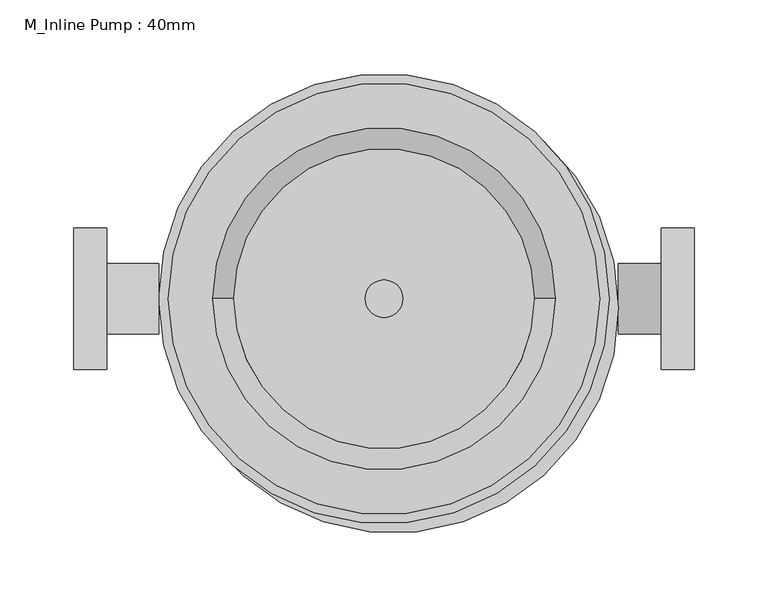
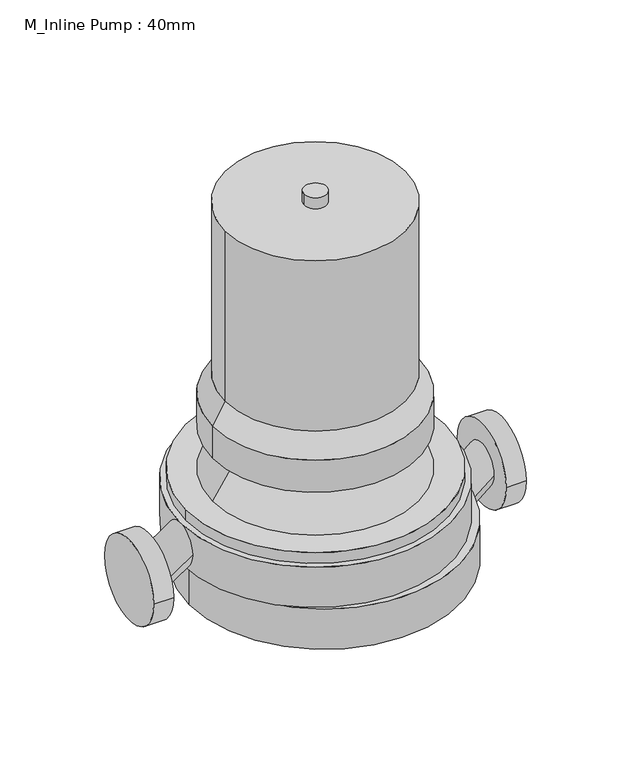
"""IFC4 building model written with IfcOpenShell, lengths in millimetres: proxy geometry, M_Inline Pump : 40mm."""

from ifc_helpers import new_model, si_unit, point, frame, frame_2d, origin, origin_with_axes, origin_2d, place, context, project, spatial, polyline, circle_curve, trimmed, segment, composite_curve, outline, extrude, source, transform, mapped, element, save
from ifc_brep_helpers import plane_surface, revolved_surface, extruded_surface, advanced_brep


def m_inline_pump_40mm_c178c80e(model_context):
    return source(origin(), model_context, "Body", "SolidModel", [
        advanced_brep(
        [(158.75, -24.0, -24.0), (158.75, 24.0, -24.0), (187.7, -24.0, 0.0), (187.7, 24.0, 0.0)],
        [
            (0, 1, circle_curve(frame((158.75, 0.0, -24.0), z_axis=(-1.0, 0.0, 0.0), x_axis=(0.0, 1.0, 0.0)), 24.0)),
            (1, 0, circle_curve(frame((158.75, 0.0, -24.0), z_axis=(-1.0, 0.0, 0.0), x_axis=(0.0, 1.0, 0.0)), 24.0)),
            (2, 3, circle_curve(frame((187.7, 0.0, 0.0), z_axis=(1.0, 0.0, 0.0), x_axis=(0.0, 1.0, 0.0)), 24.0)),
            (3, 2, circle_curve(frame((187.7, 0.0, 0.0), z_axis=(1.0, 0.0, 0.0), x_axis=(0.0, 1.0, 0.0)), 24.0)),
            (3, 1),
            (0, 2),
        ],
        [
            plane_surface(frame((158.75, 0.0, -24.0), z_axis=(-1.0, 0.0, 0.0), x_axis=(0.0, 0.0, -1.0))),
            plane_surface(frame((187.7, 0.0, 0.0), z_axis=(1.0, 0.0, 0.0), x_axis=(0.0, 0.0, -1.0))),
            extruded_surface(trimmed(circle_curve(frame((187.7, 0.0, 0.0), z_axis=(-1.0, 0.0, 0.0), x_axis=(0.0, 1.0, 0.0)), 24.0), [point((187.7, -24.0, 0.0))], [point((187.7, 24.0, 0.0))], True, "CARTESIAN"), (-28.94999999999999, 0.0, -24.0), 37.604554245463405),
            extruded_surface(trimmed(circle_curve(frame((187.7, 0.0, 0.0), z_axis=(-1.0, 0.0, 0.0), x_axis=(0.0, 1.0, 0.0)), 24.0), [point((187.7, 24.0, 0.0))], [point((187.7, -24.0, 0.0))], True, "CARTESIAN"), (-28.94999999999999, 0.0, -24.0), 37.604554245463405),
        ],
        [
            (0, [[1, 2]]),
            (1, [[3, 4]]),
            (2, [[-4, 5, -1, 6]]),
            (3, [[-3, -6, -2, -5]]),
        ],
    ),
        extrude(outline(composite_curve([segment(trimmed(circle_curve(origin_2d(), 48.0), [point((-48.0, 0.0))], [point((48.0, 0.0))], False, "CARTESIAN"), True, "CONTINUOUS"), segment(trimmed(circle_curve(origin_2d(), 48.0), [point((48.0, 0.0))], [point((-48.0, 0.0))], False, "CARTESIAN"), True, "CONTINUOUS")], self_intersect=False)), frame((187.7, 0.0, 0.0), z_axis=(1.0, 0.0, 0.0), x_axis=(0.0, 1.0, 0.0)), (0.0, 0.0, 1.0), 22.3),
        advanced_brep(
        [(-152.4, -24.0, 24.0), (-152.4, 24.0, 24.0), (-187.7, -24.0, 0.0), (-187.7, 24.0, 0.0)],
        [
            (0, 1, circle_curve(frame((-152.4, 0.0, 24.0), z_axis=(1.0, 0.0, 0.0), x_axis=(0.0, 1.0, 0.0)), 24.0)),
            (1, 0, circle_curve(frame((-152.4, 0.0, 24.0), z_axis=(1.0, 0.0, 0.0), x_axis=(0.0, 1.0, 0.0)), 24.0)),
            (2, 3, circle_curve(frame((-187.7, 0.0, 0.0), z_axis=(-1.0, 0.0, 0.0), x_axis=(0.0, 1.0, 0.0)), 24.0)),
            (3, 2, circle_curve(frame((-187.7, 0.0, 0.0), z_axis=(-1.0, 0.0, 0.0), x_axis=(0.0, 1.0, 0.0)), 24.0)),
            (3, 1),
            (0, 2),
        ],
        [
            plane_surface(frame((-152.4, 0.0, 24.0), z_axis=(1.0, 0.0, 0.0), x_axis=(0.0, 0.0, -1.0))),
            plane_surface(frame((-187.7, 0.0, 0.0), z_axis=(-1.0, 0.0, 0.0), x_axis=(0.0, 0.0, -1.0))),
            extruded_surface(trimmed(circle_curve(frame((-187.7, 0.0, 0.0), z_axis=(1.0, 0.0, 0.0), x_axis=(0.0, 1.0, 0.0)), 24.0), [point((-187.7, -24.0, 0.0))], [point((-187.7, 24.0, 0.0))], True, "CARTESIAN"), (35.29999999999998, 0.0, 24.0), 42.68594616498501),
            extruded_surface(trimmed(circle_curve(frame((-187.7, 0.0, 0.0), z_axis=(1.0, 0.0, 0.0), x_axis=(0.0, 1.0, 0.0)), 24.0), [point((-187.7, 24.0, 0.0))], [point((-187.7, -24.0, 0.0))], True, "CARTESIAN"), (35.29999999999998, 0.0, 24.0), 42.68594616498501),
        ],
        [
            (0, [[1, 2]]),
            (1, [[3, 4]]),
            (2, [[-4, 5, -1, 6]]),
            (3, [[-3, -6, -2, -5]]),
        ],
    ),
        extrude(outline(composite_curve([segment(trimmed(circle_curve(origin_2d(), 48.0), [point((-48.0, 0.0))], [point((48.0, 0.0))], False, "CARTESIAN"), True, "CONTINUOUS"), segment(trimmed(circle_curve(origin_2d(), 48.0), [point((48.0, 0.0))], [point((-48.0, 0.0))], False, "CARTESIAN"), True, "CONTINUOUS")], self_intersect=False)), frame((-210.0, 0.0, 0.0), z_axis=(1.0, 0.0, 0.0), x_axis=(0.0, 1.0, 0.0)), (0.0, 0.0, 1.0), 22.3),
        extrude(outline(composite_curve([segment(trimmed(circle_curve(origin_2d(), 12.7), [point((-12.7, 0.0))], [point((12.7, 0.0))], False, "CARTESIAN"), True, "CONTINUOUS"), segment(trimmed(circle_curve(origin_2d(), 12.7), [point((12.7, 0.0))], [point((-12.7, 0.0))], False, "CARTESIAN"), True, "CONTINUOUS")], self_intersect=False)), frame((0.0, 0.0, 378.0), z_axis=(0.0, 0.0, 1.0), x_axis=(1.0, 0.0, 0.0)), (0.0, 0.0, 1.0), 13.0),
        extrude(outline(composite_curve([segment(trimmed(circle_curve(origin_2d(), 152.4), [point((-152.4, 0.0))], [point((152.4, 0.0))], False, "CARTESIAN"), True, "CONTINUOUS"), segment(trimmed(circle_curve(origin_2d(), 152.4), [point((152.4, 0.0))], [point((-152.4, 0.0))], False, "CARTESIAN"), True, "CONTINUOUS")], self_intersect=False)), origin_with_axes(), (0.0, 0.0, 1.0), 48.0),
        extrude(outline(composite_curve([segment(trimmed(circle_curve(frame_2d((6.35, -6.35)), 152.4), [point((-146.05, -6.35))], [point((158.75, -6.35))], False, "CARTESIAN"), True, "CONTINUOUS"), segment(trimmed(circle_curve(frame_2d((6.35, -6.35)), 152.4), [point((158.75, -6.35))], [point((-146.05, -6.35))], False, "CARTESIAN"), True, "CONTINUOUS")], self_intersect=False)), frame((0.0, 0.0, -48.0), z_axis=(0.0, 0.0, 1.0), x_axis=(1.0, 0.0, 0.0)), (0.0, 0.0, 1.0), 48.0),
        extrude(outline(composite_curve([segment(trimmed(circle_curve(origin_2d(), 38.1), [point((-38.1, 0.0))], [point((38.1, 0.0))], False, "CARTESIAN"), True, "CONTINUOUS"), segment(trimmed(circle_curve(origin_2d(), 38.1), [point((38.1, 0.0))], [point((-38.1, 0.0))], False, "CARTESIAN"), True, "CONTINUOUS")], self_intersect=False)), frame((0.0, 0.0, -60.7198438), z_axis=(0.0, 0.0, 1.0), x_axis=(1.0, 0.0, 0.0)), (0.0, 0.0, 1.0), 12.7198438),
        extrude(outline(composite_curve([segment(trimmed(circle_curve(origin_2d(), 12.7), [point((-12.7, 0.0))], [point((12.7, 0.0))], False, "CARTESIAN"), True, "CONTINUOUS"), segment(trimmed(circle_curve(origin_2d(), 12.7), [point((12.7, 0.0))], [point((-12.7, 0.0))], False, "CARTESIAN"), True, "CONTINUOUS")], self_intersect=False)), frame((0.0, 0.0, -67.0698438), z_axis=(0.0, 0.0, 1.0), x_axis=(1.0, 0.0, 0.0)), (0.0, 0.0, 1.0), 6.35),
        extrude(outline(composite_curve([segment(trimmed(circle_curve(origin_2d(), 101.6), [point((-101.6, 0.0))], [point((101.6, 0.0))], False, "CARTESIAN"), True, "CONTINUOUS"), segment(trimmed(circle_curve(origin_2d(), 101.6), [point((101.6, 0.0))], [point((-101.6, 0.0))], False, "CARTESIAN"), True, "CONTINUOUS")], self_intersect=False)), frame((0.0, 0.0, 175.0), z_axis=(0.0, 0.0, 1.0), x_axis=(1.0, 0.0, 0.0)), (0.0, 0.0, 1.0), 203.0),
        advanced_brep(
        [(-101.6, 0.0, 175.0), (101.6, 0.0, 175.0), (-115.8875, 0.0, 150.0), (115.8875, 0.0, 150.0)],
        [
            (0, 1, circle_curve(frame((0.0, 0.0, 175.0), z_axis=(0.0, 0.0, 1.0), x_axis=(-1.0, 0.0, 0.0)), 101.6)),
            (1, 0, circle_curve(frame((0.0, 0.0, 175.0), z_axis=(0.0, 0.0, 1.0), x_axis=(1.0, 0.0, 0.0)), 101.6)),
            (2, 3, circle_curve(frame((0.0, 0.0, 150.0), z_axis=(0.0, 0.0, -1.0), x_axis=(1.0, 0.0, 0.0)), 115.8875)),
            (3, 2, circle_curve(frame((0.0, 0.0, 150.0), z_axis=(0.0, 0.0, -1.0), x_axis=(-1.0, 0.0, 0.0)), 115.8875)),
            (3, 1),
            (0, 2),
        ],
        [
            plane_surface(frame((0.0, 0.0, 175.0), z_axis=(0.0, 0.0, 1.0), x_axis=(0.0, -1.0, 0.0))),
            plane_surface(frame((0.0, 0.0, 150.0), z_axis=(0.0, 0.0, -1.0), x_axis=(0.0, -1.0, 0.0))),
            revolved_surface(polyline([(-101.60000000156576, 0.0, 175.0), (-115.8875, 0.0, 150.0)]), (0.0, 0.0, 352.7777778), (0.0, 0.0, -1.0)),
            revolved_surface(polyline([(101.60000000156576, 0.0, 175.0), (115.8875, 0.0, 150.0)]), (0.0, 0.0, 352.7777778), (0.0, 0.0, -1.0)),
        ],
        [
            (0, [[1, 2]]),
            (1, [[3, 4]]),
            (2, [[-4, 5, -1, 6]]),
            (3, [[-3, -6, -2, -5]]),
        ],
    ),
        extrude(outline(composite_curve([segment(trimmed(circle_curve(origin_2d(), 115.8875), [point((-115.8875, 0.0))], [point((115.8875, 0.0))], False, "CARTESIAN"), True, "CONTINUOUS"), segment(trimmed(circle_curve(origin_2d(), 115.8875), [point((115.8875, 0.0))], [point((-115.8875, 0.0))], False, "CARTESIAN"), True, "CONTINUOUS")], self_intersect=False)), frame((0.0, 0.0, 112.0), z_axis=(0.0, 0.0, 1.0), x_axis=(1.0, 0.0, 0.0)), (0.0, 0.0, 1.0), 38.0),
        advanced_brep(
        [(-82.55, 0.0, 112.0), (82.55, 0.0, 112.0), (-115.8875, 0.0, 61.0), (115.8875, 0.0, 61.0)],
        [
            (0, 1, circle_curve(frame((0.0, 0.0, 112.0), z_axis=(0.0, 0.0, 1.0), x_axis=(-1.0, 0.0, 0.0)), 82.55)),
            (1, 0, circle_curve(frame((0.0, 0.0, 112.0), z_axis=(0.0, 0.0, 1.0), x_axis=(1.0, 0.0, 0.0)), 82.55)),
            (2, 3, circle_curve(frame((0.0, 0.0, 61.0), z_axis=(0.0, 0.0, -1.0), x_axis=(1.0, 0.0, 0.0)), 115.8875)),
            (3, 2, circle_curve(frame((0.0, 0.0, 61.0), z_axis=(0.0, 0.0, -1.0), x_axis=(-1.0, 0.0, 0.0)), 115.8875)),
            (3, 1),
            (0, 2),
        ],
        [
            plane_surface(frame((0.0, 0.0, 112.0), z_axis=(0.0, 0.0, 1.0), x_axis=(0.0, -1.0, 0.0))),
            plane_surface(frame((0.0, 0.0, 61.0), z_axis=(0.0, 0.0, -1.0), x_axis=(0.0, -1.0, 0.0))),
            revolved_surface(polyline([(-82.55000000268635, 0.0, 111.99999999999999), (-115.8875, 0.0, 61.0)]), (0.0, 0.0, 238.2857143), (0.0, 0.0, -1.0)),
            revolved_surface(polyline([(82.55000000268635, 0.0, 111.99999999999999), (115.8875, 0.0, 61.0)]), (0.0, 0.0, 238.2857143), (0.0, 0.0, -1.0)),
        ],
        [
            (0, [[1, 2]]),
            (1, [[3, 4]]),
            (2, [[-4, 5, -1, 6]]),
            (3, [[-3, -6, -2, -5]]),
        ],
    ),
        extrude(outline(composite_curve([segment(trimmed(circle_curve(origin_2d(), 146.05), [point((-146.05, 0.0))], [point((146.05, 0.0))], False, "CARTESIAN"), True, "CONTINUOUS"), segment(trimmed(circle_curve(origin_2d(), 146.05), [point((146.05, 0.0))], [point((-146.05, 0.0))], False, "CARTESIAN"), True, "CONTINUOUS")], self_intersect=False)), frame((0.0, 0.0, 48.0), z_axis=(0.0, 0.0, 1.0), x_axis=(1.0, 0.0, 0.0)), (0.0, 0.0, 1.0), 13.0),
    ])


if __name__ == "__main__":
    model = new_model("IFC4")
    model_context = context("Model", 3, world=origin())
    ifc_project = project(units=[si_unit("LENGTHUNIT", "METRE", prefix="MILLI")], contexts=[model_context])
    site = spatial("IfcSite", under=ifc_project)
    building = spatial("IfcBuilding", under=site)
    placement = place(None, origin())
    m_inline_pump_40mm_shape = m_inline_pump_40mm_c178c80e(model_context)
    element("IfcBuildingElementProxy", 1, Name="M_Inline Pump : 40mm", ObjectType="M_Inline Pump : 40mm", at=placement, inside=building, context=model_context, shape_type="MappedRepresentation", body=[
        mapped(m_inline_pump_40mm_shape, transform((0.0, 0.0, 0.0), x_axis=(1.0, 0.0, 0.0), y_axis=(0.0, 1.0, 0.0), z_axis=(0.0, 0.0, 1.0))),
    ])
    save(model, "model.ifc")

# Revit data of these elements
# Type "M_Inline Pump : 40mm"
#   Pump Speed = "1750"
#   Voltage = 230 V
#   Suction Radius = 20 mm
#   Suction Outside Radius = 24 mm
#   Suction Outside Diameter = 48 mm
#   Suction Nominal Diameter = 40 mm
#   Suction Flange Outside Radius = 48 mm
#   Suction Flange Outside Diameter = 96 mm
#   Suction Flange Length = 22.3 mm
#   Length = 420 mm
#   Height = 48 mm
#   Half Length = 210 mm
#   Discharge Radius = 20 mm
#   Discharge Outside Radius = 24 mm
#   Discharge Outside Diameter = 48 mm
#   Discharge Nominal Diameter = 40 mm
#   Discharge Flange Outside Radius = 48 mm
#   Discharge Flange Outside Diameter = 96 mm
#   Discharge Flange Length = 22.3 mm
#   Apparent Load = 2000 VA
#   Number of Poles = 2
#   Pump Material = none
#   Load Classification = Appliance - Dwelling Unit
